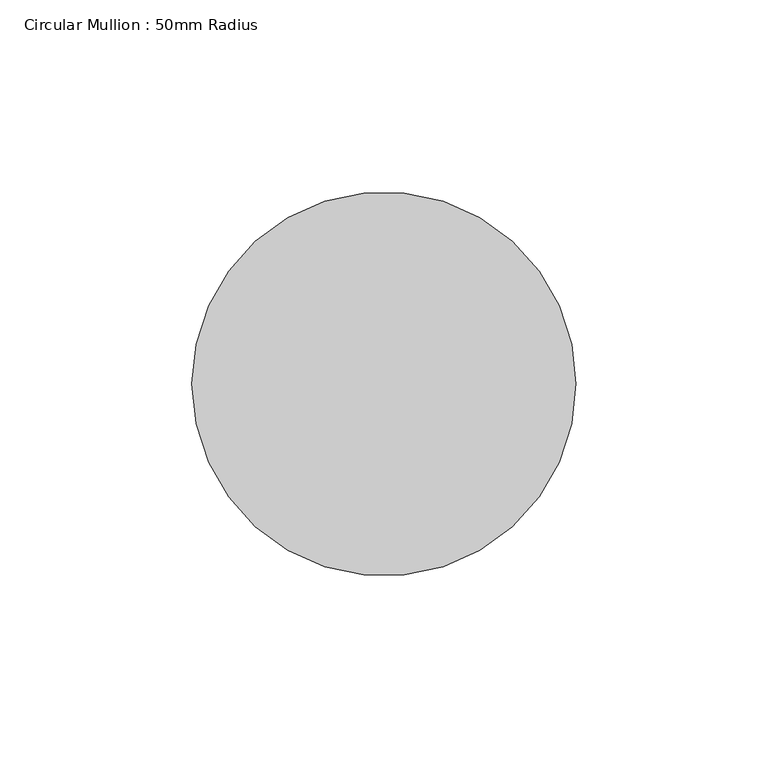
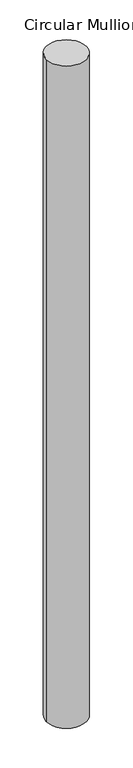
"""IFC4 building model written with IfcOpenShell, lengths in millimetres: member geometry, Circular Mullion : 50mm Radius."""

from ifc_helpers import new_model, si_unit, point, frame, frame_2d, origin, place, context, project, spatial, circle_curve, trimmed, segment, composite_curve, outline, extrude, source, transform, mapped, element, save


def circular_mullion_50mm_radius_0f4ae468(model_context):
    return source(origin(), model_context, "Body", "SweptSolid", [
        extrude(outline(composite_curve([segment(trimmed(circle_curve(frame_2d((-50.0, 0.0)), 50.0), [point((0.0, 0.0))], [point((-100.0, 0.0))], False, "CARTESIAN"), True, "CONTINUOUS"), segment(trimmed(circle_curve(frame_2d((-50.0, 0.0)), 50.0), [point((-100.0, 0.0))], [point((0.0, 0.0))], False, "CARTESIAN"), True, "CONTINUOUS")], self_intersect=False)), frame((0.0, 0.0, -1759.0343706), z_axis=(0.0, 0.0, 1.0), x_axis=(1.0, 0.0, 0.0)), (0.0, 0.0, 1.0), 1759.0343706),
    ])


if __name__ == "__main__":
    model = new_model("IFC4")
    model_context = context("Model", 3, world=origin())
    ifc_project = project(units=[si_unit("LENGTHUNIT", "METRE", prefix="MILLI")], contexts=[model_context])
    site = spatial("IfcSite", under=ifc_project)
    building = spatial("IfcBuilding", under=site)
    placement = place(None, origin())
    circular_mullion_50mm_radius_shape = circular_mullion_50mm_radius_0f4ae468(model_context)
    element("IfcMember", 1, ObjectType="Circular Mullion : 50mm Radius", at=placement, inside=building, context=model_context, shape_type="MappedRepresentation", body=[
        mapped(circular_mullion_50mm_radius_shape, transform((0.0, 0.0, 0.0), x_axis=(1.0, 0.0, 0.0), y_axis=(0.0, 1.0, 0.0), z_axis=(0.0, 0.0, 1.0))),
    ])
    save(model, "model.ifc")

# Revit data of these elements
# Type "Circular Mullion : 50mm Radius"
#   built-in parameter 1007350 = 0.164042 (stored number, unit not read)
# Element 1 (IfcMember, "Circular Mullion : 50mm Radius")
#   Materials on its faces: "Aluminium"
# Materials
#   "Aluminium": class "Metal", colour RGB 247 247 247, transparency 0, Description = "Aluminium 6061", Cost = 0
